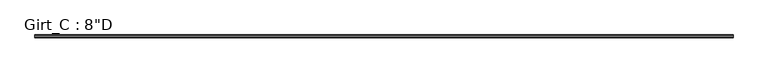
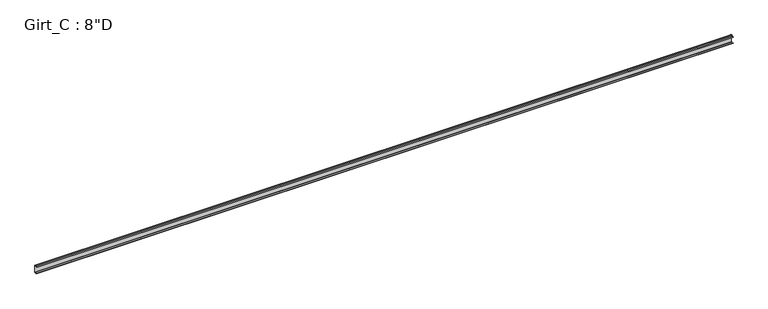
"""IFC4 building model written with IfcOpenShell, lengths in millimetres: beam geometry."""

from ifc_helpers import new_model, si_unit, point, frame, frame_2d, origin, place, context, project, spatial, polyline, circle_curve, trimmed, segment, composite_curve, outline, extrude, source, transform, mapped, element, save


def beam_3aeb7176(model_context):
    return source(origin(), model_context, "Body", "SweptSolid", [
        extrude(outline(composite_curve([segment(polyline([(-63.5, 101.6), (-3.3734375, 101.6)]), True, "CONTINUOUS"), segment(trimmed(circle_curve(frame_2d((-3.3734375, 96.8375)), 4.7625), [point((-3.3734375, 101.6))], [point((1.3890625, 96.8375))], False, "CARTESIAN"), True, "CONTINUOUS"), segment(polyline([(1.3890625, 96.8375), (1.3890625, -96.8375)]), True, "CONTINUOUS"), segment(trimmed(circle_curve(frame_2d((-3.3734375, -96.8375)), 4.7625), [point((1.3890625, -96.8375))], [point((-3.3734375, -101.6))], False, "CARTESIAN"), True, "CONTINUOUS"), segment(polyline([(-3.3734375, -101.6), (-63.5, -101.6), (-75.745104, -87.0068534), (-73.6169367, -85.221109), (-62.204539, -98.821875), (-3.2694106, -98.821875)]), True, "CONTINUOUS"), segment(trimmed(circle_curve(frame_2d((-3.3748024, -96.8389339)), 1.9857399), [point((-3.2694106, -98.821875))], [point((-1.3890625, -96.8389339))], True, "CARTESIAN"), True, "CONTINUOUS"), segment(polyline([(-1.3890625, -96.8389339), (-1.3890625, 96.8381931)]), True, "CONTINUOUS"), segment(trimmed(circle_curve(frame_2d((-3.3741066, 96.8381931)), 1.9850441), [point((-1.3890625, 96.8381931))], [point((-3.3005807, 98.821875))], True, "CARTESIAN"), True, "CONTINUOUS"), segment(polyline([(-3.3005807, 98.821875), (-62.204539, 98.821875), (-73.6169367, 85.221109), (-75.745104, 87.0068534), (-63.5, 101.6)]), True, "CONTINUOUS")], self_intersect=False)), frame((-9369.4242831, 0.0, 0.0), z_axis=(1.0, 0.0, 0.0), x_axis=(0.0, 1.0, 0.0)), (0.0, 0.0, 1.0), 18738.8485661),
    ])


if __name__ == "__main__":
    model = new_model("IFC4")
    model_context = context("Model", 3, world=origin())
    ifc_project = project(units=[si_unit("LENGTHUNIT", "METRE", prefix="MILLI")], contexts=[model_context])
    site = spatial("IfcSite", under=ifc_project)
    building = spatial("IfcBuilding", under=site)
    placement = place(None, origin())
    beam_shape = beam_3aeb7176(model_context)
    element("IfcBeam", 1, ObjectType="Girt_C : 8\"D", at=placement, inside=building, context=model_context, shape_type="MappedRepresentation", body=[
        mapped(beam_shape, transform((0.0, 0.0, 0.0), x_axis=(1.0, 0.0, 0.0), y_axis=(0.0, 1.0, 0.0), z_axis=(0.0, 0.0, 1.0))),
    ])
    save(model, "model.ifc")

# Revit data of these elements
# Type "Girt_C : 8\"D"
#   Web_Thickness = 0' - 0 7/64"
#   Length [instance default] = 10' - 0"
#   Leg_1 = 0' - 2 1/2"
#   Height = 0' - 8"
#   Structural Material [instance default] = none
